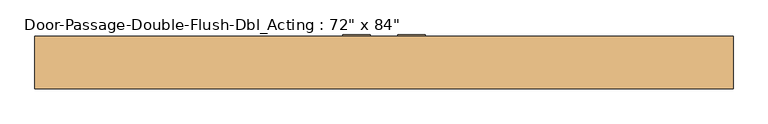
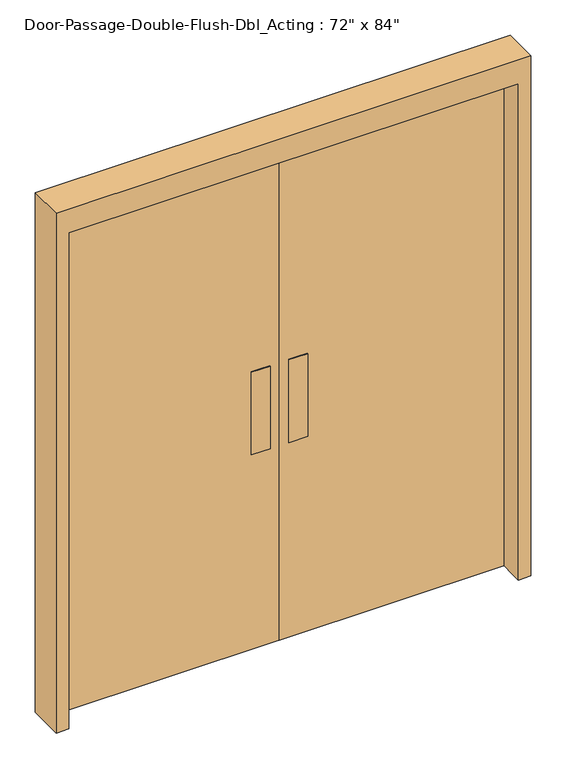
"""IFC4 building model written with IfcOpenShell, lengths in millimetres: door geometry."""

import ifcopenshell
import ifcopenshell.guid

model = None  # the IFC model being written
_history = None  # IfcOwnerHistory: only IFC2X3 demands one
_inside = {}  # id of a spatial element -> (the spatial element, [elements in it])
_under = {}  # id of a project, library or spatial element -> (it, [spatial elements below it])
_declared = {}  # id of a project -> (the project, [libraries it declares])
_typed = {}  # id of a type object -> (the type object, [elements of that type])
_made_of = {}  # id of a material, layer set ... -> (it, [elements and type objects made of it])


def new_model(schema):
    """Start an empty IFC model of exactly this schema.

    Asked for "IFC4X3", IfcOpenShell would pick the latest addendum, in which some entities
    have other attributes; the version numbers below select the first issue.
    IFC2X3 requires an IfcOwnerHistory on every rooted entity: one is made here for all.
    """
    global model, _history
    if schema == "IFC4X3":
        model = ifcopenshell.file(schema_version=(4, 3, 0, 0))
    else:
        model = ifcopenshell.file(schema=schema)
    _inside.clear()
    _under.clear()
    _declared.clear()
    _typed.clear()
    _made_of.clear()
    _history = None
    if model.schema == "IFC2X3":
        org = make("IfcOrganization", Name="unknown")
        user = make(
            "IfcPersonAndOrganization",
            ThePerson=make("IfcPerson", FamilyName="unknown"),
            TheOrganization=org,
        )
        app = make(
            "IfcApplication",
            ApplicationDeveloper=org,
            Version="unknown",
            ApplicationFullName="unknown",
            ApplicationIdentifier="unknown",
        )
        _history = make(
            "IfcOwnerHistory",
            OwningUser=user,
            OwningApplication=app,
            ChangeAction="ADDED",
            CreationDate=0,
        )
    return model


def make(cls, **values):
    """One entity of the class cls with the attributes given. An attribute that is None is left unset."""
    return model.create_entity(
        cls, **{name: value for name, value in values.items() if value is not None}
    )


def rooted(cls, **values):
    """An entity with a GlobalId (a new one), such as an element, a storey or a relation."""
    return make(cls, GlobalId=ifcopenshell.guid.new(), OwnerHistory=_history, **values)


def si_unit(unit_type, name, prefix=None):
    """IfcSIUnit, for example si_unit("LENGTHUNIT", "METRE", prefix="MILLI")."""
    return make("IfcSIUnit", UnitType=unit_type, Prefix=prefix, Name=name)


def assignment(units):
    """IfcUnitAssignment: the units of a project."""
    return None if units is None else make("IfcUnitAssignment", Units=units)


def point(xyz):
    """IfcCartesianPoint."""
    return None if xyz is None else make("IfcCartesianPoint", Coordinates=xyz)


def direction(xyz):
    """IfcDirection."""
    return None if xyz is None else make("IfcDirection", DirectionRatios=xyz)


def frame(location, z_axis=None, x_axis=None):
    """IfcAxis2Placement3D, a coordinate frame: its origin and axes. An axis left out is left unset."""
    return make(
        "IfcAxis2Placement3D",
        Location=point(location),
        Axis=direction(z_axis),
        RefDirection=direction(x_axis),
    )


def origin():
    """The frame at (0, 0, 0) with its axes left unset."""
    return frame((0.0, 0.0, 0.0))


def origin_with_axes():
    """The frame at (0, 0, 0) with the z axis (0, 0, 1) and the x axis (1, 0, 0) written out."""
    return frame((0.0, 0.0, 0.0), z_axis=(0.0, 0.0, 1.0), x_axis=(1.0, 0.0, 0.0))


def place(relative_to, where):
    """IfcLocalPlacement: puts the frame where relative to a parent placement (None: the world)."""
    return make(
        "IfcLocalPlacement", PlacementRelTo=relative_to, RelativePlacement=where
    )


def context(
    kind, dimensions, precision=None, world=None, true_north=None, identifier=None
):
    """IfcGeometricRepresentationContext, for example the 3D "Model" context."""
    return make(
        "IfcGeometricRepresentationContext",
        ContextIdentifier=identifier,
        ContextType=kind,
        CoordinateSpaceDimension=dimensions,
        Precision=precision,
        WorldCoordinateSystem=world,
        TrueNorth=true_north,
    )


def project(units=None, contexts=None):
    """IfcProject with its units and contexts."""
    return rooted(
        "IfcProject",
        Name="project",
        RepresentationContexts=contexts,
        UnitsInContext=assignment(units),
    )


def spatial(cls, under=None, at=None, **own):
    """A site, building, storey or space (cls), placed at a placement, below another one or the project."""
    s = rooted(cls, ObjectPlacement=at, **own)
    if under is not None:
        _under.setdefault(under.id(), (under, []))[1].append(s)
    return s


def polyline(points):
    """IfcPolyline through the points."""
    return make("IfcPolyline", Points=[point(p) for p in points])


def outline(outer, holes=None, kind="AREA"):
    """IfcArbitraryClosedProfileDef: a profile drawn as a closed curve; with holes, ...WithVoids."""
    if holes is None:
        return make("IfcArbitraryClosedProfileDef", ProfileType=kind, OuterCurve=outer)
    return make(
        "IfcArbitraryProfileDefWithVoids",
        ProfileType=kind,
        OuterCurve=outer,
        InnerCurves=holes,
    )


def extrude(swept, where, along, depth):
    """IfcExtrudedAreaSolid: the profile swept, set in the frame where, extruded along a direction by depth."""
    return make(
        "IfcExtrudedAreaSolid",
        SweptArea=swept,
        Position=where,
        ExtrudedDirection=direction(along),
        Depth=depth,
    )


def shape(context_of_items, identifier, shape_type, items):
    """IfcShapeRepresentation: the items that make up one representation, for example the "Body"."""
    return make(
        "IfcShapeRepresentation",
        ContextOfItems=context_of_items,
        RepresentationIdentifier=identifier,
        RepresentationType=shape_type,
        Items=items,
    )


def source(mapping_origin, context_of_items, identifier, shape_type, items):
    """IfcRepresentationMap: a shape defined once, which mapped items show again and again."""
    return make(
        "IfcRepresentationMap",
        MappingOrigin=mapping_origin,
        MappedRepresentation=shape(context_of_items, identifier, shape_type, items),
    )


def transform(
    local_origin,
    x_axis=None,
    y_axis=None,
    z_axis=None,
    scale=None,
    scale2=None,
    scale3=None,
    uniform=True,
):
    """IfcCartesianTransformationOperator3D, or its non-uniform kind. x_axis, y_axis, z_axis: its Axis1, 2, 3."""
    if uniform:
        return make(
            "IfcCartesianTransformationOperator3D",
            Axis1=direction(x_axis),
            Axis2=direction(y_axis),
            LocalOrigin=point(local_origin),
            Scale=scale,
            Axis3=direction(z_axis),
        )
    return make(
        "IfcCartesianTransformationOperator3DnonUniform",
        Axis1=direction(x_axis),
        Axis2=direction(y_axis),
        LocalOrigin=point(local_origin),
        Scale=scale,
        Axis3=direction(z_axis),
        Scale2=scale2,
        Scale3=scale3,
    )


def mapped(mapping_source, mapping_target):
    """IfcMappedItem: shows the shape of a source again, moved by a transform."""
    return make(
        "IfcMappedItem", MappingSource=mapping_source, MappingTarget=mapping_target
    )


def made_of(thing, what):
    """Note that an element or type object is made of a material, layer set ...; save() writes the relation."""
    if what is not None:
        _made_of.setdefault(what.id(), (what, []))[1].append(thing)
    return thing


def element(
    cls,
    number,
    at=None,
    inside=None,
    cuts=None,
    type_object=None,
    material=None,
    context=None,
    identifier="Body",
    shape_type=None,
    held_by="IfcProductDefinitionShape",
    body=None,
    shapes=None,
    **own,
):
    """One element of the class cls, such as IfcWall. Its Tag is "e" and its number.

    at: its placement. inside: the storey or other place that contains it. cuts: it is an
    opening in that element (IfcRelVoidsElement). A single representation is given by context,
    identifier, shape_type and body (its items); several are given by shapes. held_by: the class
    of the entity that holds the representations. save() writes the other relations.
    """
    e = rooted(cls, Tag="e%d" % number, ObjectPlacement=at, **own)
    if body is not None:
        shapes = [shape(context, identifier, shape_type, body)]
    if shapes is not None:
        e.Representation = make(held_by, Representations=shapes)
    if inside is not None:
        _inside.setdefault(inside.id(), (inside, []))[1].append(e)
    if cuts is not None:
        rooted(
            "IfcRelVoidsElement", RelatingBuildingElement=cuts, RelatedOpeningElement=e
        )
    if type_object is not None:
        _typed.setdefault(type_object.id(), (type_object, []))[1].append(e)
    return made_of(e, material)


def aggregate(whole, parts):
    """IfcRelAggregates: a whole, such as a stair, and the parts it consists of."""
    return rooted("IfcRelAggregates", RelatingObject=whole, RelatedObjects=parts)


def save(model, path):
    """Write the relations noted so far, then the file.

    IfcRelAggregates (storeys below a building ...), IfcRelContainedInSpatialStructure (elements
    in a storey), IfcRelDefinesByType, IfcRelAssociatesMaterial and IfcRelDeclares: one each for
    every whole, place, type object, material and project.
    """
    for whole, parts in _under.values():
        aggregate(whole, parts)
    for where, things in _inside.values():
        rooted(
            "IfcRelContainedInSpatialStructure",
            RelatedElements=things,
            RelatingStructure=where,
        )
    for kind, things in _typed.values():
        rooted("IfcRelDefinesByType", RelatedObjects=things, RelatingType=kind)
    for what, things in _made_of.values():
        rooted("IfcRelAssociatesMaterial", RelatedObjects=things, RelatingMaterial=what)
    for by, libraries in _declared.values():
        rooted("IfcRelDeclares", RelatingContext=by, RelatedDefinitions=libraries)
    model.write(path)


def door_d44e9ae0(model_context):
    return source(origin(), model_context, "Body", "SweptSolid", [
        extrude(outline(polyline([(-38.1, 34.925), (-114.3, 34.925), (-114.3, 38.1), (-38.1, 38.1), (-38.1, 34.925)])), frame((0.0, 0.0, 838.2), z_axis=(0.0, 0.0, 1.0), x_axis=(1.0, 0.0, 0.0)), (0.0, 0.0, 1.0), 355.6),
        extrude(outline(polyline([(-38.1, 85.725), (-38.1, 82.55), (-114.3, 82.55), (-114.3, 85.725), (-38.1, 85.725)])), frame((0.0, 0.0, 838.2), z_axis=(0.0, 0.0, 1.0), x_axis=(1.0, 0.0, 0.0)), (0.0, 0.0, 1.0), 355.6),
        extrude(outline(polyline([(38.1, 34.925), (38.1, 38.1), (114.3, 38.1), (114.3, 34.925), (38.1, 34.925)])), frame((0.0, 0.0, 838.2), z_axis=(0.0, 0.0, 1.0), x_axis=(1.0, 0.0, 0.0)), (0.0, 0.0, 1.0), 355.6),
        extrude(outline(polyline([(38.1, 85.725), (114.3, 85.725), (114.3, 82.55), (38.1, 82.55), (38.1, 85.725)])), frame((0.0, 0.0, 838.2), z_axis=(0.0, 0.0, 1.0), x_axis=(1.0, 0.0, 0.0)), (0.0, 0.0, 1.0), 355.6),
        extrude(outline(polyline([(0.0, 914.4), (0.0, 965.2), (2235.2, 965.2), (2235.2, -965.2), (0.0, -965.2), (0.0, -914.4), (2133.6, -914.4), (2133.6, 914.4), (0.0, 914.4)])), frame((0.0, -63.5, 0.0), z_axis=(0.0, 1.0, 0.0), x_axis=(0.0, 0.0, 1.0)), (0.0, 0.0, 1.0), 146.05),
        extrude(outline(polyline([(914.4, 38.1), (1.5875, 38.1), (1.5875, 82.55), (914.4, 82.55), (914.4, 38.1)])), origin_with_axes(), (0.0, 0.0, 1.0), 2133.6),
        extrude(outline(polyline([(-1.5875, 38.1), (-914.4, 38.1), (-914.4, 82.55), (-1.5875, 82.55), (-1.5875, 38.1)])), origin_with_axes(), (0.0, 0.0, 1.0), 2133.6),
    ])


if __name__ == "__main__":
    model = new_model("IFC4")
    model_context = context("Model", 3, world=origin())
    ifc_project = project(units=[si_unit("LENGTHUNIT", "METRE", prefix="MILLI")], contexts=[model_context])
    site = spatial("IfcSite", under=ifc_project)
    building = spatial("IfcBuilding", under=site)
    placement = place(None, origin())
    door_shape = door_d44e9ae0(model_context)
    element("IfcDoor", 1, ObjectType="Door-Passage-Double-Flush-Dbl_Acting : 72\" x 84\"", at=placement, inside=building, context=model_context, shape_type="MappedRepresentation", body=[
        mapped(door_shape, transform((0.0, 0.0, 0.0), x_axis=(1.0, 0.0, 0.0), y_axis=(0.0, 1.0, 0.0), z_axis=(0.0, 0.0, 1.0))),
    ])
    save(model, "model.ifc")

# Revit data of these elements
# Type "Door-Passage-Double-Flush-Dbl_Acting : 72\" x 84\""
#   Type Mark = "22"
#   Assembly Code = "B2030200"
#   Analytic Construction = "Metal"
#   W = 3' - 0"
#   Thickness = 0' - 1 3/4"
#   Thermal Resistance (R) = 1.5338 (h·ft²·°F)/BTU
#   Swing Angle [instance default] = 90.00°
#   Strike Height = 3' - 4"
#   Single Panel Width = 3' - 0"
#   Rough Width [instance default] = 6' - 4"
#   Rough Height [instance default] = 7' - 4"
#   MF Opening Height [instance default] = 0' - 4"
#   MF Opening Width [instance default] = 0' - 4"
#   Inset Calculate [instance default] = 0' - 4"
#   Masonry Inset [instance default] = 0' - 1"
#   Height = 7' - 0"
#   Width = 6' - 0"
#   Heat Transfer Coefficient (U) = 0.6520 BTU/(h·ft²·°F)
#   Masonry Frame Depth = 0' - 5 3/4"
#   Masonry Frame [instance default] = yes
#   Function = 1
#   Dry Wall Frame [instance default] = no
#   Panel Material = Metal - Paint Finish - Brindle
#   Frame Material = Metal - Paint Finish - Grey
#   Door Handle Material = Aluminium
#   Visual Light Transmittance = 0
#   Solar Heat Gain Coefficient = 0
#   Wall Closure = (empty or 0)
# Element 1 (IfcDoor, "Door-Passage-Double-Flush-Dbl_Acting : 72\" x 84\"")
#   Materials on its faces: "Aluminium", "Metal - Paint Finish - Grey", "Metal - Paint Finish - Brindle"
# Materials
#   "Metal - Paint Finish - Brindle": class "Paint", colour RGB 164 133 98, transparency 0, Cost = 0
#   "Metal - Paint Finish - Grey": class "Paint", colour RGB 104 104 104, transparency 0, Cost = 0
#   "Aluminium": class "Metal", colour RGB 244 244 244, transparency 0, Description = "Aluminum 6061", Cost = 0
